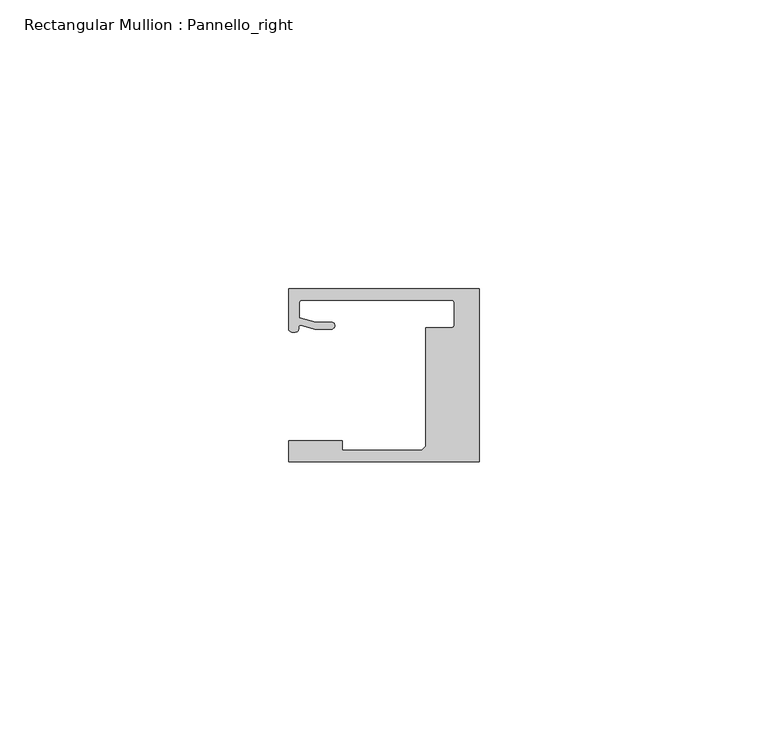
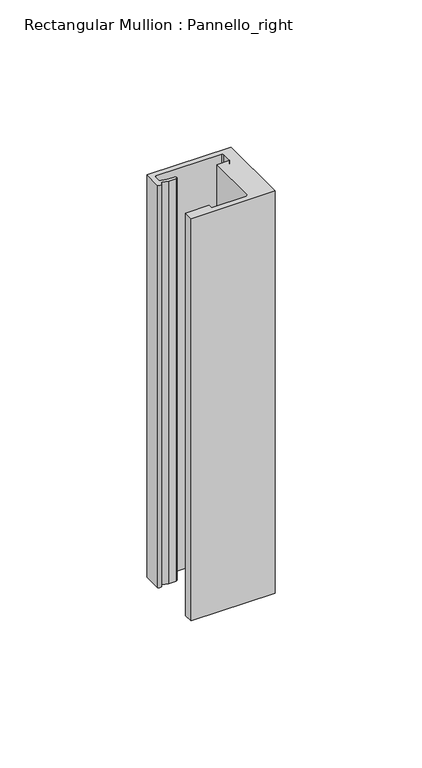
"""IFC4 building model written with IfcOpenShell, lengths in millimetres: member geometry, Rectangular Mullion : Pannello_right."""

import ifcopenshell
import ifcopenshell.guid

model = None  # the IFC model being written
_history = None  # IfcOwnerHistory: only IFC2X3 demands one
_inside = {}  # id of a spatial element -> (the spatial element, [elements in it])
_under = {}  # id of a project, library or spatial element -> (it, [spatial elements below it])
_declared = {}  # id of a project -> (the project, [libraries it declares])
_typed = {}  # id of a type object -> (the type object, [elements of that type])
_made_of = {}  # id of a material, layer set ... -> (it, [elements and type objects made of it])


def new_model(schema):
    """Start an empty IFC model of exactly this schema.

    Asked for "IFC4X3", IfcOpenShell would pick the latest addendum, in which some entities
    have other attributes; the version numbers below select the first issue.
    IFC2X3 requires an IfcOwnerHistory on every rooted entity: one is made here for all.
    """
    global model, _history
    if schema == "IFC4X3":
        model = ifcopenshell.file(schema_version=(4, 3, 0, 0))
    else:
        model = ifcopenshell.file(schema=schema)
    _inside.clear()
    _under.clear()
    _declared.clear()
    _typed.clear()
    _made_of.clear()
    _history = None
    if model.schema == "IFC2X3":
        org = make("IfcOrganization", Name="unknown")
        user = make(
            "IfcPersonAndOrganization",
            ThePerson=make("IfcPerson", FamilyName="unknown"),
            TheOrganization=org,
        )
        app = make(
            "IfcApplication",
            ApplicationDeveloper=org,
            Version="unknown",
            ApplicationFullName="unknown",
            ApplicationIdentifier="unknown",
        )
        _history = make(
            "IfcOwnerHistory",
            OwningUser=user,
            OwningApplication=app,
            ChangeAction="ADDED",
            CreationDate=0,
        )
    return model


def make(cls, **values):
    """One entity of the class cls with the attributes given. An attribute that is None is left unset."""
    return model.create_entity(
        cls, **{name: value for name, value in values.items() if value is not None}
    )


def rooted(cls, **values):
    """An entity with a GlobalId (a new one), such as an element, a storey or a relation."""
    return make(cls, GlobalId=ifcopenshell.guid.new(), OwnerHistory=_history, **values)


def si_unit(unit_type, name, prefix=None):
    """IfcSIUnit, for example si_unit("LENGTHUNIT", "METRE", prefix="MILLI")."""
    return make("IfcSIUnit", UnitType=unit_type, Prefix=prefix, Name=name)


def assignment(units):
    """IfcUnitAssignment: the units of a project."""
    return None if units is None else make("IfcUnitAssignment", Units=units)


def point(xyz):
    """IfcCartesianPoint."""
    return None if xyz is None else make("IfcCartesianPoint", Coordinates=xyz)


def direction(xyz):
    """IfcDirection."""
    return None if xyz is None else make("IfcDirection", DirectionRatios=xyz)


def frame(location, z_axis=None, x_axis=None):
    """IfcAxis2Placement3D, a coordinate frame: its origin and axes. An axis left out is left unset."""
    return make(
        "IfcAxis2Placement3D",
        Location=point(location),
        Axis=direction(z_axis),
        RefDirection=direction(x_axis),
    )


def origin():
    """The frame at (0, 0, 0) with its axes left unset."""
    return frame((0.0, 0.0, 0.0))


def place(relative_to, where):
    """IfcLocalPlacement: puts the frame where relative to a parent placement (None: the world)."""
    return make(
        "IfcLocalPlacement", PlacementRelTo=relative_to, RelativePlacement=where
    )


def context(
    kind, dimensions, precision=None, world=None, true_north=None, identifier=None
):
    """IfcGeometricRepresentationContext, for example the 3D "Model" context."""
    return make(
        "IfcGeometricRepresentationContext",
        ContextIdentifier=identifier,
        ContextType=kind,
        CoordinateSpaceDimension=dimensions,
        Precision=precision,
        WorldCoordinateSystem=world,
        TrueNorth=true_north,
    )


def project(units=None, contexts=None):
    """IfcProject with its units and contexts."""
    return rooted(
        "IfcProject",
        Name="project",
        RepresentationContexts=contexts,
        UnitsInContext=assignment(units),
    )


def spatial(cls, under=None, at=None, **own):
    """A site, building, storey or space (cls), placed at a placement, below another one or the project."""
    s = rooted(cls, ObjectPlacement=at, **own)
    if under is not None:
        _under.setdefault(under.id(), (under, []))[1].append(s)
    return s


def polyline(points):
    """IfcPolyline through the points."""
    return make("IfcPolyline", Points=[point(p) for p in points])


def circle_curve(where, radius):
    """IfcCircle in the frame where."""
    return make("IfcCircle", Position=where, Radius=radius)


def shape(context_of_items, identifier, shape_type, items):
    """IfcShapeRepresentation: the items that make up one representation, for example the "Body"."""
    return make(
        "IfcShapeRepresentation",
        ContextOfItems=context_of_items,
        RepresentationIdentifier=identifier,
        RepresentationType=shape_type,
        Items=items,
    )


def source(mapping_origin, context_of_items, identifier, shape_type, items):
    """IfcRepresentationMap: a shape defined once, which mapped items show again and again."""
    return make(
        "IfcRepresentationMap",
        MappingOrigin=mapping_origin,
        MappedRepresentation=shape(context_of_items, identifier, shape_type, items),
    )


def transform(
    local_origin,
    x_axis=None,
    y_axis=None,
    z_axis=None,
    scale=None,
    scale2=None,
    scale3=None,
    uniform=True,
):
    """IfcCartesianTransformationOperator3D, or its non-uniform kind. x_axis, y_axis, z_axis: its Axis1, 2, 3."""
    if uniform:
        return make(
            "IfcCartesianTransformationOperator3D",
            Axis1=direction(x_axis),
            Axis2=direction(y_axis),
            LocalOrigin=point(local_origin),
            Scale=scale,
            Axis3=direction(z_axis),
        )
    return make(
        "IfcCartesianTransformationOperator3DnonUniform",
        Axis1=direction(x_axis),
        Axis2=direction(y_axis),
        LocalOrigin=point(local_origin),
        Scale=scale,
        Axis3=direction(z_axis),
        Scale2=scale2,
        Scale3=scale3,
    )


def mapped(mapping_source, mapping_target):
    """IfcMappedItem: shows the shape of a source again, moved by a transform."""
    return make(
        "IfcMappedItem", MappingSource=mapping_source, MappingTarget=mapping_target
    )


def made_of(thing, what):
    """Note that an element or type object is made of a material, layer set ...; save() writes the relation."""
    if what is not None:
        _made_of.setdefault(what.id(), (what, []))[1].append(thing)
    return thing


def element(
    cls,
    number,
    at=None,
    inside=None,
    cuts=None,
    type_object=None,
    material=None,
    context=None,
    identifier="Body",
    shape_type=None,
    held_by="IfcProductDefinitionShape",
    body=None,
    shapes=None,
    **own,
):
    """One element of the class cls, such as IfcWall. Its Tag is "e" and its number.

    at: its placement. inside: the storey or other place that contains it. cuts: it is an
    opening in that element (IfcRelVoidsElement). A single representation is given by context,
    identifier, shape_type and body (its items); several are given by shapes. held_by: the class
    of the entity that holds the representations. save() writes the other relations.
    """
    e = rooted(cls, Tag="e%d" % number, ObjectPlacement=at, **own)
    if body is not None:
        shapes = [shape(context, identifier, shape_type, body)]
    if shapes is not None:
        e.Representation = make(held_by, Representations=shapes)
    if inside is not None:
        _inside.setdefault(inside.id(), (inside, []))[1].append(e)
    if cuts is not None:
        rooted(
            "IfcRelVoidsElement", RelatingBuildingElement=cuts, RelatedOpeningElement=e
        )
    if type_object is not None:
        _typed.setdefault(type_object.id(), (type_object, []))[1].append(e)
    return made_of(e, material)


def aggregate(whole, parts):
    """IfcRelAggregates: a whole, such as a stair, and the parts it consists of."""
    return rooted("IfcRelAggregates", RelatingObject=whole, RelatedObjects=parts)


def save(model, path):
    """Write the relations noted so far, then the file.

    IfcRelAggregates (storeys below a building ...), IfcRelContainedInSpatialStructure (elements
    in a storey), IfcRelDefinesByType, IfcRelAssociatesMaterial and IfcRelDeclares: one each for
    every whole, place, type object, material and project.
    """
    for whole, parts in _under.values():
        aggregate(whole, parts)
    for where, things in _inside.values():
        rooted(
            "IfcRelContainedInSpatialStructure",
            RelatedElements=things,
            RelatingStructure=where,
        )
    for kind, things in _typed.values():
        rooted("IfcRelDefinesByType", RelatedObjects=things, RelatingType=kind)
    for what, things in _made_of.values():
        rooted("IfcRelAssociatesMaterial", RelatedObjects=things, RelatingMaterial=what)
    for by, libraries in _declared.values():
        rooted("IfcRelDeclares", RelatingContext=by, RelatedDefinitions=libraries)
    model.write(path)


def plane_surface(at):
    """IfcPlane: the flat surface through the origin of the frame at, square to its z axis."""
    return make("IfcPlane", Position=at)


def cylinder_surface(at, radius):
    """IfcCylindricalSurface: all points at the distance radius from the z axis of the frame at."""
    return make("IfcCylindricalSurface", Position=at, Radius=radius)


def revolved_surface(curve, axis_point, axis_direction):
    """IfcSurfaceOfRevolution: the curve turned about the line through axis_point along axis_direction."""
    return make(
        "IfcSurfaceOfRevolution",
        SweptCurve=make("IfcArbitraryOpenProfileDef", ProfileType="CURVE", Curve=curve),
        AxisPosition=make("IfcAxis1Placement", Location=point(axis_point), Axis=direction(axis_direction)),
    )


def extruded_surface(curve, direction_of_extrusion, depth):
    """IfcSurfaceOfLinearExtrusion: the curve pushed along a direction by depth."""
    return make(
        "IfcSurfaceOfLinearExtrusion",
        SweptCurve=make("IfcArbitraryOpenProfileDef", ProfileType="CURVE", Curve=curve),
        ExtrudedDirection=direction(direction_of_extrusion),
        Depth=depth,
    )


def spline_curve(degree, points, multiplicities, knots, weights=None):
    """IfcBSplineCurveWithKnots; with weights, IfcRationalBSplineCurveWithKnots."""
    own = dict(
        Degree=degree,
        ControlPointsList=[point(p) for p in points],
        CurveForm="UNSPECIFIED",
        ClosedCurve=False,
        SelfIntersect=False,
        KnotMultiplicities=multiplicities,
        Knots=knots,
        KnotSpec="UNSPECIFIED",
    )
    if weights is None:
        return make("IfcBSplineCurveWithKnots", **own)
    return make("IfcRationalBSplineCurveWithKnots", WeightsData=weights, **own)


def advanced_brep(points, edges, surfaces, faces):
    """IfcAdvancedBrep: a solid bounded by faces that lie on surfaces and meet in shared edges.

    An edge is (start, end): straight between two places in points (the first is 0);
    or (start, end, curve); or (start, end, curve, False) where it runs against its curve.
    A face is (place in surfaces, loops), or (place, loops, False) where it looks against
    its surface's normal. A loop lists edges by number (the first is 1), with a minus sign
    where the edge is run from its end to its start. The first loop is the outer one.
    """
    corners = [point(p) for p in points]
    vertices = [make("IfcVertexPoint", VertexGeometry=c) for c in corners]
    made = []
    for start, end, *more in edges:
        made.append(
            make(
                "IfcEdgeCurve",
                EdgeStart=vertices[start],
                EdgeEnd=vertices[end],
                EdgeGeometry=more[0] if more else make("IfcPolyline", Points=[corners[start], corners[end]]),
                SameSense=more[1] if len(more) > 1 else True,
            )
        )
    hull = []
    for where, loops, *sense in faces:
        bounds = []
        for j, loop in enumerate(loops):
            ring = [make("IfcOrientedEdge", EdgeElement=made[abs(k) - 1], Orientation=k > 0) for k in loop]
            bounds.append(
                make(
                    "IfcFaceOuterBound" if j == 0 else "IfcFaceBound",
                    Bound=make("IfcEdgeLoop", EdgeList=ring),
                    Orientation=True,
                )
            )
        hull.append(make("IfcAdvancedFace", Bounds=bounds, FaceSurface=surfaces[where], SameSense=sense[0] if sense else True))
    return make("IfcAdvancedBrep", Outer=make("IfcClosedShell", CfsFaces=hull))


def rectangular_mullion_pannello_right_08fec6ed(model_context):
    return source(origin(), model_context, "Body", "AdvancedBrep", [
        advanced_brep(
        [(-33.0, -15.0, 0.0), (0.0, -15.0, 0.0), (0.0, 15.0, 0.0), (-33.0000135, 15.0, 0.0), (-33.0000135, 8.0000472, 0.0), (-30.9223017, 8.6490241, 0.0), (-28.4999305, 7.9999523, 0.0), (-25.59998, 7.9999523, 0.0), (-25.59998, 9.1999523, 0.0), (-28.3419477, 9.1999523, 0.0), (-31.19998, 9.9657591, 0.0), (-31.19998, 12.50001, 0.0), (-30.69998, 13.00001, 0.0), (-4.7999726, 13.00001, 0.0), (-4.2999726, 12.50001, 0.0), (-4.2999726, 8.7500595, 0.0), (-4.7999726, 8.2500595, 0.0), (-9.2999726, 8.2500595, 0.0), (-9.2999726, -12.2999849, 0.0), (-10.0000103, -13.0000004, 0.0), (-23.700041, -13.0000004, 0.0), (-23.700041, -11.3000004, 0.0), (-33.0, -11.3000004, 0.0), (-33.0, -15.0, -166.9999865), (-33.0, -11.3000004, -166.9999865), (-23.700041, -11.3000004, -166.9999865), (-23.700041, -13.0000004, -166.9999865), (-10.0000103, -13.0000004, -166.9999865), (-9.2999726, -12.2999849, -166.9999865), (-9.2999726, 8.2500595, -166.9999865), (-4.7999726, 8.2500595, -166.9999865), (-4.2999726, 8.7500595, -166.9999865), (-4.2999726, 12.50001, -166.9999865), (-4.7999726, 13.00001, -166.9999865), (-30.69998, 13.00001, -166.9999865), (-31.19998, 12.50001, -166.9999865), (-31.19998, 9.9657591, -166.9999865), (-28.3419477, 9.1999523, -166.9999865), (-25.59998, 9.1999523, -166.9999865), (-25.59998, 7.9999523, -166.9999865), (-28.4999305, 7.9999523, -166.9999865), (-30.9223017, 8.6490241, -166.9999865), (-33.0000135, 8.0000472, -166.9999865), (-33.0000135, 15.0, -166.9999865), (0.0, 15.0, -166.9999865), (0.0, -15.0, -166.9999865)],
        [
            (0, 1),
            (1, 2),
            (2, 3),
            (3, 4),
            (4, 5, spline_curve(3, [(-33.0000135, 8.0000472, 0.0), (-33.0000135, 7.457047519, 0.0), (-32.262327879, 7.456527435, 0.0), (-31.357433266, 7.563996614, 0.0), (-31.305645054, 7.690065204, 0.0), (-31.298563602, 8.366228555, 0.0), (-31.312054066, 8.717747958, 0.0), (-30.9223017, 8.6490241, 0.0)], [4, 2, 2, 4], [0.0, 0.0027053965905959043, 0.0058611956533709, 0.007702013405570312])),
            (5, 6),
            (6, 7),
            (7, 8, circle_curve(frame((-25.59998, 8.5999523, 0.0), z_axis=(0.0, 0.0, 1.0), x_axis=(0.0, 1.0, 0.0)), 0.6)),
            (8, 9),
            (9, 10),
            (10, 11),
            (11, 12, circle_curve(frame((-30.69998, 12.50001, 0.0), z_axis=(0.0, 0.0, -1.0), x_axis=(0.0, 1.0, 0.0)), 0.5)),
            (12, 13),
            (13, 14, circle_curve(frame((-4.7999726, 12.50001, 0.0), z_axis=(0.0, 0.0, -1.0), x_axis=(1.0, 0.0, 0.0)), 0.5)),
            (14, 15),
            (15, 16, circle_curve(frame((-4.7999726, 8.7500595, 0.0), z_axis=(0.0, 0.0, -1.0), x_axis=(0.0, -1.0, 0.0)), 0.5)),
            (16, 17),
            (17, 18),
            (18, 19),
            (19, 20),
            (20, 21),
            (21, 22),
            (22, 0),
            (23, 24),
            (24, 25),
            (25, 26),
            (26, 27),
            (27, 28),
            (28, 29),
            (29, 30),
            (30, 31, circle_curve(frame((-4.7999726, 8.7500595, -166.9999865), z_axis=(0.0, 0.0, 1.0), x_axis=(0.0, -1.0, 0.0)), 0.5)),
            (31, 32),
            (32, 33, circle_curve(frame((-4.7999726, 12.50001, -166.9999865), z_axis=(0.0, 0.0, 1.0), x_axis=(1.0, 0.0, 0.0)), 0.5)),
            (33, 34),
            (34, 35, circle_curve(frame((-30.69998, 12.50001, -166.9999865), z_axis=(0.0, 0.0, 1.0), x_axis=(0.0, 1.0, 0.0)), 0.5)),
            (35, 36),
            (36, 37),
            (37, 38),
            (38, 39, circle_curve(frame((-25.59998, 8.5999523, -166.9999865), z_axis=(0.0, 0.0, -1.0), x_axis=(0.0, 1.0, 0.0)), 0.6)),
            (39, 40),
            (40, 41),
            (41, 42, spline_curve(3, [(-30.9223017, 8.6490241, -166.9999865), (-31.312054066, 8.717747958, -166.9999865), (-31.298563602, 8.366228555, -166.9999865), (-31.305645054, 7.690065204, -166.9999865), (-31.357433266, 7.563996614, -166.9999865), (-32.262327879, 7.456527435, -166.9999865), (-33.0000135, 7.457047519, -166.9999865), (-33.0000135, 8.0000472, -166.9999865)], [4, 2, 2, 4], [0.0, 0.001840817752199412, 0.004996616814974408, 0.007702013405570312])),
            (42, 43),
            (43, 44),
            (44, 45),
            (45, 23),
            (0, 23),
            (45, 1),
            (44, 2),
            (43, 3),
            (42, 4),
            (41, 5),
            (40, 6),
            (39, 7),
            (38, 8),
            (37, 9),
            (36, 10),
            (35, 11),
            (34, 12),
            (33, 13),
            (32, 14),
            (31, 15),
            (30, 16),
            (29, 17),
            (28, 18),
            (27, 19),
            (26, 20),
            (25, 21),
            (24, 22),
        ],
        [
            plane_surface(frame((0.0, -36.2491502, 0.0), z_axis=(0.0, 0.0, 1.0), x_axis=(-1.0, 0.0, 0.0))),
            plane_surface(frame((0.0, -36.2491502, -166.9999865), z_axis=(0.0, 0.0, -1.0), x_axis=(-1.0, 0.0, 0.0))),
            plane_surface(frame((-33.0, -15.0, 0.0), z_axis=(0.0, -1.0, 0.0), x_axis=(0.0, 0.0, -1.0))),
            plane_surface(frame((0.0, -15.0, 0.0), z_axis=(1.0, 0.0, 0.0), x_axis=(0.0, 0.0, -1.0))),
            plane_surface(frame((0.0, 15.0, 0.0), z_axis=(0.0, 1.0, 0.0), x_axis=(0.0, 0.0, -1.0))),
            plane_surface(frame((-33.0000135, 15.0, 0.0), z_axis=(-1.0, 0.0, 0.0), x_axis=(0.0, 0.0, -1.0))),
            extruded_surface(spline_curve(3, [(-33.0000135, 8.0000472, -166.9999865), (-33.0000135, 7.457047519, -166.9999865), (-32.262327879, 7.456527435, -166.9999865), (-31.357433266, 7.563996614, -166.9999865), (-31.305645054, 7.690065204, -166.9999865), (-31.298563602, 8.366228555, -166.9999865), (-31.312054066, 8.717747958, -166.9999865), (-30.9223017, 8.6490241, -166.9999865)], [4, 2, 2, 4], [0.0, 0.0027053965905959043, 0.0058611956533709, 0.007702013405570312]), (0.0, 0.0, 166.9999865), 166.9999865),
            plane_surface(frame((-30.9223017, 8.6490241, 0.0), z_axis=(-0.2588188320019168, -0.965925883389178, 0.0), x_axis=(0.0, 0.0, -1.0))),
            plane_surface(frame((-28.4999305, 7.9999523, 0.0), z_axis=(0.0, -1.0, 0.0), x_axis=(0.0, 0.0, -1.0))),
            cylinder_surface(frame((-25.59998, 8.5999523, 0.0), z_axis=(0.0, 0.0, 1.0), x_axis=(0.0, 1.0, 0.0)), 0.6),
            plane_surface(frame((-25.59998, 9.1999523, 0.0), z_axis=(0.0, 1.0, 0.0), x_axis=(0.0, 0.0, -1.0))),
            plane_surface(frame((-28.3419477, 9.1999523, 0.0), z_axis=(0.2588188320428738, 0.9659258833782035, 0.0), x_axis=(0.0, 0.0, -1.0))),
            plane_surface(frame((-31.19998, 9.9657591, 0.0), z_axis=(1.0, 0.0, 0.0), x_axis=(0.0, 0.0, -1.0))),
            revolved_surface(polyline([(-30.69998, 13.00001, -166.9999865), (-30.69998, 13.00001, 0.0)]), (-30.69998, 12.50001, 0.0), (0.0, 0.0, -1.0)),
            plane_surface(frame((-30.69998, 13.00001, 0.0), z_axis=(0.0, -1.0, 0.0), x_axis=(0.0, 0.0, -1.0))),
            revolved_surface(polyline([(-4.2999726, 12.50001, -166.9999865), (-4.2999726, 12.50001, 0.0)]), (-4.7999726, 12.50001, 0.0), (0.0, 0.0, -1.0)),
            plane_surface(frame((-4.2999726, 12.50001, 0.0), z_axis=(-1.0, 0.0, 0.0), x_axis=(0.0, 0.0, -1.0))),
            revolved_surface(polyline([(-4.7999726, 8.2500595, -166.9999865), (-4.7999726, 8.2500595, 0.0)]), (-4.7999726, 8.7500595, 0.0), (0.0, 0.0, -1.0)),
            plane_surface(frame((-4.7999726, 8.2500595, 0.0), z_axis=(0.0, 1.0, 0.0), x_axis=(0.0, 0.0, -1.0))),
            plane_surface(frame((-9.2999726, 8.2500595, 0.0), z_axis=(-1.0, 0.0, 0.0), x_axis=(0.0, 0.0, -1.0))),
            plane_surface(frame((-9.2999726, -12.2999849, 0.0), z_axis=(-0.7070955486278075, 0.7071180135668587, 0.0), x_axis=(0.0, 0.0, -1.0))),
            plane_surface(frame((-10.0000103, -13.0000004, 0.0), z_axis=(0.0, 1.0, 0.0), x_axis=(0.0, 0.0, -1.0))),
            plane_surface(frame((-23.700041, -13.0000004, 0.0), z_axis=(1.0, 0.0, 0.0), x_axis=(0.0, 0.0, -1.0))),
            plane_surface(frame((-23.700041, -11.3000004, 0.0), z_axis=(0.0, 1.0, 0.0), x_axis=(0.0, 0.0, -1.0))),
            plane_surface(frame((-33.0, -11.3000004, 0.0), z_axis=(-1.0, 0.0, 0.0), x_axis=(0.0, 0.0, -1.0))),
        ],
        [
            (0, [[1, 2, 3, 4, 5, 6, 7, 8, 9, 10, 11, 12, 13, 14, 15, 16, 17, 18, 19, 20, 21, 22, 23]]),
            (1, [[24, 25, 26, 27, 28, 29, 30, 31, 32, 33, 34, 35, 36, 37, 38, 39, 40, 41, 42, 43, 44, 45, 46]]),
            (2, [[-1, 47, -46, 48]]),
            (3, [[-2, -48, -45, 49]]),
            (4, [[-3, -49, -44, 50]]),
            (5, [[-4, -50, -43, 51]]),
            (6, [[-5, -51, -42, 52]]),
            (7, [[-6, -52, -41, 53]]),
            (8, [[-7, -53, -40, 54]]),
            (9, [[-8, -54, -39, 55]]),
            (10, [[-9, -55, -38, 56]]),
            (11, [[-10, -56, -37, 57]]),
            (12, [[-11, -57, -36, 58]]),
            (13, [[-12, -58, -35, 59]]),
            (14, [[-13, -59, -34, 60]]),
            (15, [[-14, -60, -33, 61]]),
            (16, [[-15, -61, -32, 62]]),
            (17, [[-16, -62, -31, 63]]),
            (18, [[-17, -63, -30, 64]]),
            (19, [[-18, -64, -29, 65]]),
            (20, [[-19, -65, -28, 66]]),
            (21, [[-20, -66, -27, 67]]),
            (22, [[-21, -67, -26, 68]]),
            (23, [[-22, -68, -25, 69]]),
            (24, [[-23, -69, -24, -47]]),
        ],
    ),
    ])


if __name__ == "__main__":
    model = new_model("IFC4")
    model_context = context("Model", 3, world=origin())
    ifc_project = project(units=[si_unit("LENGTHUNIT", "METRE", prefix="MILLI")], contexts=[model_context])
    site = spatial("IfcSite", under=ifc_project)
    building = spatial("IfcBuilding", under=site)
    placement = place(None, origin())
    rectangular_mullion_pannello_right_shape = rectangular_mullion_pannello_right_08fec6ed(model_context)
    element("IfcMember", 1, ObjectType="Rectangular Mullion : Pannello_right", at=placement, inside=building, context=model_context, shape_type="MappedRepresentation", body=[
        mapped(rectangular_mullion_pannello_right_shape, transform((0.0, 0.0, 0.0), x_axis=(1.0, 0.0, 0.0), y_axis=(0.0, 1.0, 0.0), z_axis=(0.0, 0.0, 1.0))),
    ])
    save(model, "model.ifc")

# Revit data of these elements
# Type "Rectangular Mullion : Pannello_right"
#   built-in parameter 1007322 = 0.0984252 (stored number, unit not read)
#   built-in parameter 1007321 = 0.0305117 (stored number, unit not read)
#   built-in parameter 1007320 = 0 (stored number, unit not read)
